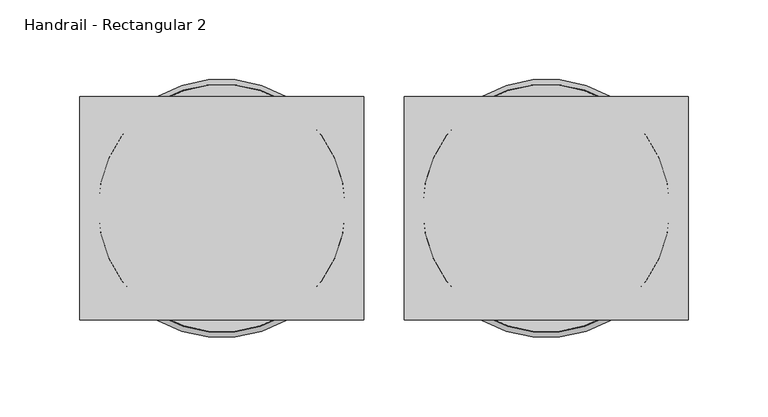
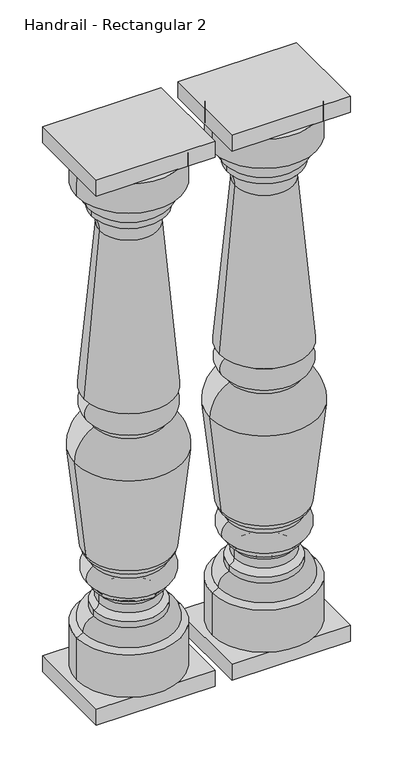
"""IFC4 building model written with IfcOpenShell, lengths in millimetres: railing geometry, Handrail - Rectangular 2."""

from ifc_helpers import new_model, si_unit, point, frame, origin, place, context, project, spatial, polyline, circle_curve, ellipse_curve, trimmed, outline, extrude, source, transform, mapped, element, save
from ifc_brep_helpers import plane_surface, cylinder_surface, revolved_surface, advanced_brep


def handrail_rectangular_2_8120b437(model_context):
    return source(origin(), model_context, "Body", "SolidModel", [
        advanced_brep(
        [(9662.0521895, -1691.0164768, 949.325), (9584.4909506, -1691.0164768, 949.325), (9739.6134284, -1691.0164768, 949.325), (9739.8396895, -1691.0164768, 136.525), (9584.2646895, -1691.0164768, 136.525), (9662.0521895, -1691.0164768, 136.525), (9739.8396895, -1691.0164768, 203.2), (9584.2646895, -1691.0164768, 203.2), (9730.2276556, -1691.0164768, 208.348485), (9593.8767235, -1691.0164768, 208.348485), (9714.4396895, -1691.0164768, 228.7310532), (9609.6646895, -1691.0164768, 228.7310532), (9714.4396895, -1691.0164768, 238.125), (9609.6646895, -1691.0164768, 238.125), (9706.8209727, -1691.0164768, 247.1598162), (9617.2834064, -1691.0164768, 247.1598162), (9706.8209727, -1691.0164768, 260.8401838), (9617.2834064, -1691.0164768, 260.8401838), (9714.4396895, -1691.0164768, 269.875), (9609.6646895, -1691.0164768, 269.875), (9714.4396895, -1691.0164768, 276.225), (9609.6646895, -1691.0164768, 276.225), (9715.2334395, -1691.0164768, 307.975), (9608.8709395, -1691.0164768, 307.975), (9715.2334395, -1691.0164768, 314.325), (9608.8709395, -1691.0164768, 314.325), (9726.0062243, -1691.0164768, 327.0157842), (9598.0981547, -1691.0164768, 327.0157842), (9743.093305, -1691.0164768, 481.3725887), (9581.0110741, -1691.0164768, 481.3725887), (9714.4396895, -1691.0164768, 528.6375), (9609.6646895, -1691.0164768, 528.6375), (9714.4396895, -1691.0164768, 534.9875), (9609.6646895, -1691.0164768, 534.9875), (9717.6146895, -1691.0164768, 569.9125), (9606.4896895, -1691.0164768, 569.9125), (9717.6146895, -1691.0164768, 573.0875), (9606.4896895, -1691.0164768, 573.0875), (9728.7271895, -1691.0164768, 577.85), (9595.3771895, -1691.0164768, 577.85), (9705.5486775, -1691.0164768, 836.3199218), (9618.5557016, -1691.0164768, 836.3199218), (9717.6146895, -1691.0164768, 863.6), (9606.4896895, -1691.0164768, 863.6), (9717.6146895, -1691.0164768, 873.125), (9606.4896895, -1691.0164768, 873.125), (9728.7271895, -1691.0164768, 900.1125), (9595.3771895, -1691.0164768, 900.1125), (9739.8396895, -1691.0164768, 903.2875), (9584.2646895, -1691.0164768, 903.2875)],
        [
            (0, 1),
            (1, 2, circle_curve(frame((9662.0521895, -1691.0164768, 949.325), z_axis=(0.0, 0.0, 1.0), x_axis=(-1.0, 0.0, 0.0)), 77.5612389)),
            (2, 0),
            (2, 1, circle_curve(frame((9662.0521895, -1691.0164768, 949.325), z_axis=(0.0, 0.0, 1.0), x_axis=(-1.0, 0.0, 0.0)), 77.5612389)),
            (3, 4, circle_curve(frame((9662.0521895, -1691.0164768, 136.525), z_axis=(0.0, 0.0, -1.0), x_axis=(-1.0, 0.0, 0.0)), 77.7875)),
            (4, 5),
            (5, 3),
            (4, 3, circle_curve(frame((9662.0521895, -1691.0164768, 136.525), z_axis=(0.0, 0.0, -1.0), x_axis=(-1.0, 0.0, 0.0)), 77.7875)),
            (6, 7, circle_curve(frame((9662.0521895, -1691.0164768, 203.2), z_axis=(0.0, 0.0, -1.0), x_axis=(-1.0, 0.0, 0.0)), 77.7875)),
            (7, 4),
            (3, 6),
            (7, 6, circle_curve(frame((9662.0521895, -1691.0164768, 203.2), z_axis=(0.0, 0.0, -1.0), x_axis=(-1.0, 0.0, 0.0)), 77.7875)),
            (8, 9, circle_curve(frame((9662.0521895, -1691.0164768, 208.348485), z_axis=(0.0, 0.0, -1.0), x_axis=(-1.0, 0.0, 0.0)), 68.175466)),
            (9, 7),
            (6, 8),
            (9, 8, circle_curve(frame((9662.0521895, -1691.0164768, 208.348485), z_axis=(0.0, 0.0, -1.0), x_axis=(-1.0, 0.0, 0.0)), 68.175466)),
            (10, 11, circle_curve(frame((9662.0521895, -1691.0164768, 228.7310532), z_axis=(0.0, 0.0, -1.0), x_axis=(-1.0, 0.0, 0.0)), 52.3875)),
            (11, 9, circle_curve(frame((9612.0397784, -1691.0164768, 210.5855331), z_axis=(0.0, -1.0, 0.0), x_axis=(1.0, 0.0, 0.0)), 18.3002991)),
            (8, 10, circle_curve(frame((9712.0646007, -1691.0164768, 210.5855331), z_axis=(0.0, -1.0, 0.0), x_axis=(-1.0, 0.0, 0.0)), 18.3002991)),
            (11, 10, circle_curve(frame((9662.0521895, -1691.0164768, 228.7310532), z_axis=(0.0, 0.0, -1.0), x_axis=(-1.0, 0.0, 0.0)), 52.3875)),
            (12, 13, circle_curve(frame((9662.0521895, -1691.0164768, 238.125), z_axis=(0.0, 0.0, -1.0), x_axis=(-1.0, 0.0, 0.0)), 52.3875)),
            (13, 11),
            (10, 12),
            (13, 12, circle_curve(frame((9662.0521895, -1691.0164768, 238.125), z_axis=(0.0, 0.0, -1.0), x_axis=(-1.0, 0.0, 0.0)), 52.3875)),
            (14, 15, circle_curve(frame((9662.0521895, -1691.0164768, 247.1598162), z_axis=(0.0, 0.0, -1.0), x_axis=(-1.0, 0.0, 0.0)), 44.7687831)),
            (15, 13, circle_curve(frame((9607.8793543, -1691.0164768, 247.3602005), z_axis=(0.0, 1.0, 0.0), x_axis=(1.0, 0.0, 0.0)), 9.4061868)),
            (12, 14, circle_curve(frame((9716.2250248, -1691.0164768, 247.3602005), z_axis=(0.0, 1.0, 0.0), x_axis=(-1.0, 0.0, 0.0)), 9.4061868)),
            (15, 14, circle_curve(frame((9662.0521895, -1691.0164768, 247.1598162), z_axis=(0.0, 0.0, -1.0), x_axis=(-1.0, 0.0, 0.0)), 44.7687831)),
            (16, 17, circle_curve(frame((9662.0521895, -1691.0164768, 260.8401838), z_axis=(0.0, 0.0, -1.0), x_axis=(-1.0, 0.0, 0.0)), 44.7687831)),
            (17, 15),
            (14, 16),
            (17, 16, circle_curve(frame((9662.0521895, -1691.0164768, 260.8401838), z_axis=(0.0, 0.0, -1.0), x_axis=(-1.0, 0.0, 0.0)), 44.7687831)),
            (18, 19, circle_curve(frame((9662.0521895, -1691.0164768, 269.875), z_axis=(0.0, 0.0, -1.0), x_axis=(-1.0, 0.0, 0.0)), 52.3875)),
            (19, 17, circle_curve(frame((9607.8793543, -1691.0164768, 260.6397995), z_axis=(0.0, 1.0, 0.0), x_axis=(1.0, 0.0, 0.0)), 9.4061868)),
            (16, 18, circle_curve(frame((9716.2250248, -1691.0164768, 260.6397995), z_axis=(0.0, 1.0, 0.0), x_axis=(-1.0, 0.0, 0.0)), 9.4061868)),
            (19, 18, circle_curve(frame((9662.0521895, -1691.0164768, 269.875), z_axis=(0.0, 0.0, -1.0), x_axis=(-1.0, 0.0, 0.0)), 52.3875)),
            (20, 21, circle_curve(frame((9662.0521895, -1691.0164768, 276.225), z_axis=(0.0, 0.0, -1.0), x_axis=(-1.0, 0.0, 0.0)), 52.3875)),
            (21, 19),
            (18, 20),
            (21, 20, circle_curve(frame((9662.0521895, -1691.0164768, 276.225), z_axis=(0.0, 0.0, -1.0), x_axis=(-1.0, 0.0, 0.0)), 52.3875)),
            (22, 23, circle_curve(frame((9662.0521895, -1691.0164768, 307.975), z_axis=(0.0, 0.0, -1.0), x_axis=(-1.0, 0.0, 0.0)), 53.18125)),
            (23, 21, circle_curve(frame((9615.2437772, -1691.0164768, 292.2493991), z_axis=(0.0, -1.0, 0.0), x_axis=(1.0, 0.0, 0.0)), 16.9678397)),
            (20, 22, circle_curve(frame((9708.8606019, -1691.0164768, 292.2493991), z_axis=(0.0, -1.0, 0.0), x_axis=(-1.0, 0.0, 0.0)), 16.9678397)),
            (23, 22, circle_curve(frame((9662.0521895, -1691.0164768, 307.975), z_axis=(0.0, 0.0, -1.0), x_axis=(-1.0, 0.0, 0.0)), 53.18125)),
            (24, 25, circle_curve(frame((9662.0521895, -1691.0164768, 314.325), z_axis=(0.0, 0.0, -1.0), x_axis=(-1.0, 0.0, 0.0)), 53.18125)),
            (25, 23),
            (22, 24),
            (25, 24, circle_curve(frame((9662.0521895, -1691.0164768, 314.325), z_axis=(0.0, 0.0, -1.0), x_axis=(-1.0, 0.0, 0.0)), 53.18125)),
            (26, 27, circle_curve(frame((9662.0521895, -1691.0164768, 327.0157842), z_axis=(0.0, 0.0, -1.0), x_axis=(-1.0, 0.0, 0.0)), 63.9540348)),
            (27, 25, circle_curve(frame((9618.704312, -1691.0164768, 333.5899445), z_axis=(0.0, -1.0, 0.0), x_axis=(1.0, 0.0, 0.0)), 21.6294545)),
            (24, 26, circle_curve(frame((9705.4000671, -1691.0164768, 333.5899445), z_axis=(0.0, -1.0, 0.0), x_axis=(-1.0, 0.0, 0.0)), 21.6294545)),
            (27, 26, circle_curve(frame((9662.0521895, -1691.0164768, 327.0157842), z_axis=(0.0, 0.0, -1.0), x_axis=(-1.0, 0.0, 0.0)), 63.9540348)),
            (28, 29, circle_curve(frame((9662.0521895, -1691.0164768, 481.3725887), z_axis=(0.0, 0.0, -1.0), x_axis=(-1.0, 0.0, 0.0)), 81.0411154)),
            (29, 27, circle_curve(frame((11075.3385198, -1691.0164768, 568.6683698), z_axis=(0.0, -1.0, 0.0), x_axis=(1.0, 0.0, 0.0)), 1496.8751012)),
            (26, 28, circle_curve(frame((8248.7658592, -1691.0164768, 568.6683698), z_axis=(0.0, -1.0, 0.0), x_axis=(-1.0, 0.0, 0.0)), 1496.8751012)),
            (29, 28, circle_curve(frame((9662.0521895, -1691.0164768, 481.3725887), z_axis=(0.0, 0.0, -1.0), x_axis=(-1.0, 0.0, 0.0)), 81.0411154)),
            (30, 31, circle_curve(frame((9662.0521895, -1691.0164768, 528.6375), z_axis=(0.0, 0.0, -1.0), x_axis=(-1.0, 0.0, 0.0)), 52.3875)),
            (31, 29, circle_curve(frame((9632.7638402, -1691.0164768, 482.3161407), z_axis=(0.0, -1.0, 0.0), x_axis=(1.0, 0.0, 0.0)), 51.7613668)),
            (28, 30, circle_curve(frame((9691.3405389, -1691.0164768, 482.3161407), z_axis=(0.0, -1.0, 0.0), x_axis=(-1.0, 0.0, 0.0)), 51.7613668)),
            (31, 30, circle_curve(frame((9662.0521895, -1691.0164768, 528.6375), z_axis=(0.0, 0.0, -1.0), x_axis=(-1.0, 0.0, 0.0)), 52.3875)),
            (32, 33, circle_curve(frame((9662.0521895, -1691.0164768, 534.9875), z_axis=(0.0, 0.0, -1.0), x_axis=(-1.0, 0.0, 0.0)), 52.3875)),
            (33, 31),
            (30, 32),
            (33, 32, circle_curve(frame((9662.0521895, -1691.0164768, 534.9875), z_axis=(0.0, 0.0, -1.0), x_axis=(-1.0, 0.0, 0.0)), 52.3875)),
            (34, 35, circle_curve(frame((9662.0521895, -1691.0164768, 569.9125), z_axis=(0.0, 0.0, -1.0), x_axis=(-1.0, 0.0, 0.0)), 55.5625)),
            (35, 33, circle_curve(frame((9614.7309419, -1691.0164768, 553.0548866), z_axis=(0.0, -1.0, 0.0), x_axis=(1.0, 0.0, 0.0)), 18.7642578)),
            (32, 34, circle_curve(frame((9709.3734372, -1691.0164768, 553.0548866), z_axis=(0.0, -1.0, 0.0), x_axis=(-1.0, 0.0, 0.0)), 18.7642578)),
            (35, 34, circle_curve(frame((9662.0521895, -1691.0164768, 569.9125), z_axis=(0.0, 0.0, -1.0), x_axis=(-1.0, 0.0, 0.0)), 55.5625)),
            (36, 37, circle_curve(frame((9662.0521895, -1691.0164768, 573.0875), z_axis=(0.0, 0.0, -1.0), x_axis=(-1.0, 0.0, 0.0)), 55.5625)),
            (37, 35),
            (34, 36),
            (37, 36, circle_curve(frame((9662.0521895, -1691.0164768, 573.0875), z_axis=(0.0, 0.0, -1.0), x_axis=(-1.0, 0.0, 0.0)), 55.5625)),
            (38, 39, circle_curve(frame((9662.0521895, -1691.0164768, 577.85), z_axis=(0.0, 0.0, -1.0), x_axis=(-1.0, 0.0, 0.0)), 66.675)),
            (39, 37),
            (36, 38),
            (39, 38, circle_curve(frame((9662.0521895, -1691.0164768, 577.85), z_axis=(0.0, 0.0, -1.0), x_axis=(-1.0, 0.0, 0.0)), 66.675)),
            (40, 41, circle_curve(frame((9662.0521895, -1691.0164768, 836.3199218), z_axis=(0.0, 0.0, -1.0), x_axis=(-1.0, 0.0, 0.0)), 43.4964879)),
            (41, 39, circle_curve(frame((7971.7192757, -1691.0164768, 853.7271544), z_axis=(0.0, 1.0, 0.0), x_axis=(1.0, 0.0, 0.0)), 1646.9284215)),
            (38, 40, circle_curve(frame((11352.3851034, -1691.0164768, 853.7271544), z_axis=(0.0, 1.0, 0.0), x_axis=(-1.0, 0.0, 0.0)), 1646.9284215)),
            (41, 40, circle_curve(frame((9662.0521895, -1691.0164768, 836.3199218), z_axis=(0.0, 0.0, -1.0), x_axis=(-1.0, 0.0, 0.0)), 43.4964879)),
            (42, 43, circle_curve(frame((9662.0521895, -1691.0164768, 863.6), z_axis=(0.0, 0.0, -1.0), x_axis=(-1.0, 0.0, 0.0)), 55.5625)),
            (43, 41, circle_curve(frame((9585.8515427, -1691.0164768, 838.1632773), z_axis=(0.0, 1.0, 0.0), x_axis=(1.0, 0.0, 0.0)), 32.7560676)),
            (40, 42, circle_curve(frame((9738.2528363, -1691.0164768, 838.1632773), z_axis=(0.0, 1.0, 0.0), x_axis=(-1.0, 0.0, 0.0)), 32.7560676)),
            (43, 42, circle_curve(frame((9662.0521895, -1691.0164768, 863.6), z_axis=(0.0, 0.0, -1.0), x_axis=(-1.0, 0.0, 0.0)), 55.5625)),
            (44, 45, circle_curve(frame((9662.0521895, -1691.0164768, 873.125), z_axis=(0.0, 0.0, -1.0), x_axis=(-1.0, 0.0, 0.0)), 55.5625)),
            (45, 43),
            (42, 44),
            (45, 44, circle_curve(frame((9662.0521895, -1691.0164768, 873.125), z_axis=(0.0, 0.0, -1.0), x_axis=(-1.0, 0.0, 0.0)), 55.5625)),
            (46, 47, circle_curve(frame((9662.0521895, -1691.0164768, 900.1125), z_axis=(0.0, 0.0, -1.0), x_axis=(-1.0, 0.0, 0.0)), 66.675)),
            (47, 45, circle_curve(frame((9624.7374113, -1691.0164768, 896.4203854), z_axis=(0.0, -1.0, 0.0), x_axis=(1.0, 0.0, 0.0)), 29.5914571)),
            (44, 46, circle_curve(frame((9699.3669678, -1691.0164768, 896.4203854), z_axis=(0.0, -1.0, 0.0), x_axis=(-1.0, 0.0, 0.0)), 29.5914571)),
            (47, 46, circle_curve(frame((9662.0521895, -1691.0164768, 900.1125), z_axis=(0.0, 0.0, -1.0), x_axis=(-1.0, 0.0, 0.0)), 66.675)),
            (48, 49, circle_curve(frame((9662.0521895, -1691.0164768, 903.2875), z_axis=(0.0, 0.0, -1.0), x_axis=(-1.0, 0.0, 0.0)), 77.7875)),
            (49, 47),
            (46, 48),
            (49, 48, circle_curve(frame((9662.0521895, -1691.0164768, 903.2875), z_axis=(0.0, 0.0, -1.0), x_axis=(-1.0, 0.0, 0.0)), 77.7875)),
            (1, 49),
            (48, 2),
        ],
        [
            plane_surface(frame((9662.0521895, -1691.0164768, 949.325), z_axis=(0.0, 0.0, 1.0), x_axis=(-1.0, 0.0, 0.0))),
            plane_surface(frame((9662.0521895, -1691.0164768, 136.525), z_axis=(0.0, 0.0, -1.0), x_axis=(-1.0, 0.0, 0.0))),
            cylinder_surface(frame((9662.0521895, -1691.0164768, 1019.175), z_axis=(0.0, 0.0, 1.0), x_axis=(-1.0, 0.0, 0.0)), 77.7875),
            revolved_surface(polyline([(9584.2646895, -1691.0164768, 203.2), (9593.8767235, -1691.0164768, 208.348485)]), (9662.0521895, -1691.0164768, 1019.175), (0.0, 0.0, 1.0)),
            revolved_surface(trimmed(ellipse_curve(frame((9612.0397784, -1691.0164768, 210.5855331), z_axis=(0.0, 1.0, 0.0), x_axis=(1.0, 0.0, 0.0)), 18.3002991, 18.3002991), [point((9593.8767235, -1691.0164768, 208.348485))], [point((9609.6646895, -1691.0164768, 228.7310532))], True, "CARTESIAN"), (9662.0521895, -1691.0164768, 1019.175), (0.0, 0.0, 1.0)),
            cylinder_surface(frame((9662.0521895, -1691.0164768, 1019.175), z_axis=(0.0, 0.0, 1.0), x_axis=(-1.0, 0.0, 0.0)), 52.3875),
            revolved_surface(trimmed(ellipse_curve(frame((9607.8793543, -1691.0164768, 247.3602005), z_axis=(0.0, -1.0, 0.0), x_axis=(1.0, 0.0, 0.0)), 9.4061868, 9.4061868), [point((9609.6646895, -1691.0164768, 238.125))], [point((9617.2834064, -1691.0164768, 247.1598162))], True, "CARTESIAN"), (9662.0521895, -1691.0164768, 1019.175), (0.0, 0.0, 1.0)),
            cylinder_surface(frame((9662.0521895, -1691.0164768, 1019.175), z_axis=(0.0, 0.0, 1.0), x_axis=(-1.0, 0.0, 0.0)), 44.7687831),
            revolved_surface(trimmed(ellipse_curve(frame((9607.8793543, -1691.0164768, 260.6397995), z_axis=(0.0, -1.0, 0.0), x_axis=(1.0, 0.0, 0.0)), 9.4061868, 9.4061868), [point((9617.2834064, -1691.0164768, 260.8401838))], [point((9609.6646895, -1691.0164768, 269.875))], True, "CARTESIAN"), (9662.0521895, -1691.0164768, 1019.175), (0.0, 0.0, 1.0)),
            revolved_surface(trimmed(ellipse_curve(frame((9615.2437772, -1691.0164768, 292.2493991), z_axis=(0.0, 1.0, 0.0), x_axis=(1.0, 0.0, 0.0)), 16.9678397, 16.9678397), [point((9609.6646895, -1691.0164768, 276.225))], [point((9608.8709395, -1691.0164768, 307.975))], True, "CARTESIAN"), (9662.0521895, -1691.0164768, 1019.175), (0.0, 0.0, 1.0)),
            cylinder_surface(frame((9662.0521895, -1691.0164768, 1019.175), z_axis=(0.0, 0.0, 1.0), x_axis=(-1.0, 0.0, 0.0)), 53.18125),
            revolved_surface(trimmed(ellipse_curve(frame((9618.704312, -1691.0164768, 333.5899445), z_axis=(0.0, 1.0, 0.0), x_axis=(1.0, 0.0, 0.0)), 21.6294545, 21.6294545), [point((9608.8709395, -1691.0164768, 314.325))], [point((9598.0981547, -1691.0164768, 327.0157842))], True, "CARTESIAN"), (9662.0521895, -1691.0164768, 1019.175), (0.0, 0.0, 1.0)),
            revolved_surface(trimmed(ellipse_curve(frame((11075.3385198, -1691.0164768, 568.6683698), z_axis=(0.0, 1.0, 0.0), x_axis=(1.0, 0.0, 0.0)), 1496.8751012, 1496.8751012), [point((9598.0981547, -1691.0164768, 327.0157842))], [point((9581.0110741, -1691.0164768, 481.3725887))], True, "CARTESIAN"), (9662.0521895, -1691.0164768, 1019.175), (0.0, 0.0, 1.0)),
            revolved_surface(trimmed(ellipse_curve(frame((9632.7638402, -1691.0164768, 482.3161407), z_axis=(0.0, 1.0, 0.0), x_axis=(1.0, 0.0, 0.0)), 51.7613668, 51.7613668), [point((9581.0110741, -1691.0164768, 481.3725887))], [point((9609.6646895, -1691.0164768, 528.6375))], True, "CARTESIAN"), (9662.0521895, -1691.0164768, 1019.175), (0.0, 0.0, 1.0)),
            revolved_surface(trimmed(ellipse_curve(frame((9614.7309419, -1691.0164768, 553.0548866), z_axis=(0.0, 1.0, 0.0), x_axis=(1.0, 0.0, 0.0)), 18.7642578, 18.7642578), [point((9609.6646895, -1691.0164768, 534.9875))], [point((9606.4896895, -1691.0164768, 569.9125))], True, "CARTESIAN"), (9662.0521895, -1691.0164768, 1019.175), (0.0, 0.0, 1.0)),
            cylinder_surface(frame((9662.0521895, -1691.0164768, 1019.175), z_axis=(0.0, 0.0, 1.0), x_axis=(-1.0, 0.0, 0.0)), 55.5625),
            revolved_surface(polyline([(9606.4896895, -1691.0164768, 573.0875), (9595.3771895, -1691.0164768, 577.85)]), (9662.0521895, -1691.0164768, 1019.175), (0.0, 0.0, 1.0)),
            revolved_surface(trimmed(ellipse_curve(frame((7971.7192757, -1691.0164768, 853.7271544), z_axis=(0.0, -1.0, 0.0), x_axis=(1.0, 0.0, 0.0)), 1646.9284215, 1646.9284215), [point((9595.3771895, -1691.0164768, 577.85))], [point((9618.5557016, -1691.0164768, 836.3199218))], True, "CARTESIAN"), (9662.0521895, -1691.0164768, 1019.175), (0.0, 0.0, 1.0)),
            revolved_surface(trimmed(ellipse_curve(frame((9585.8515427, -1691.0164768, 838.1632773), z_axis=(0.0, -1.0, 0.0), x_axis=(1.0, 0.0, 0.0)), 32.7560676, 32.7560676), [point((9618.5557016, -1691.0164768, 836.3199218))], [point((9606.4896895, -1691.0164768, 863.6))], True, "CARTESIAN"), (9662.0521895, -1691.0164768, 1019.175), (0.0, 0.0, 1.0)),
            revolved_surface(trimmed(ellipse_curve(frame((9624.7374113, -1691.0164768, 896.4203854), z_axis=(0.0, 1.0, 0.0), x_axis=(1.0, 0.0, 0.0)), 29.5914571, 29.5914571), [point((9606.4896895, -1691.0164768, 873.125))], [point((9595.3771895, -1691.0164768, 900.1125))], True, "CARTESIAN"), (9662.0521895, -1691.0164768, 1019.175), (0.0, 0.0, 1.0)),
            revolved_surface(polyline([(9595.3771895, -1691.0164768, 900.1125), (9584.2646895, -1691.0164768, 903.2875)]), (9662.0521895, -1691.0164768, 1019.175), (0.0, 0.0, 1.0)),
            revolved_surface(polyline([(9584.2646895, -1691.0164768, 903.2875), (9584.4909506, -1691.0164768, 949.325)]), (9662.0521895, -1691.0164768, 1019.175), (0.0, 0.0, 1.0)),
        ],
        [
            (0, [[1, 2, 3]]),
            (0, [[-3, 4, -1]]),
            (1, [[5, 6, 7]]),
            (1, [[8, -7, -6]]),
            (2, [[9, 10, -5, 11]]),
            (2, [[12, -11, -8, -10]]),
            (3, [[13, 14, -9, 15]]),
            (3, [[16, -15, -12, -14]]),
            (4, [[17, 18, -13, 19]]),
            (4, [[20, -19, -16, -18]]),
            (5, [[21, 22, -17, 23]]),
            (5, [[24, -23, -20, -22]]),
            (6, [[25, 26, -21, 27]]),
            (6, [[28, -27, -24, -26]]),
            (7, [[29, 30, -25, 31]]),
            (7, [[32, -31, -28, -30]]),
            (8, [[33, 34, -29, 35]]),
            (8, [[36, -35, -32, -34]]),
            (5, [[37, 38, -33, 39]]),
            (5, [[40, -39, -36, -38]]),
            (9, [[41, 42, -37, 43]]),
            (9, [[44, -43, -40, -42]]),
            (10, [[45, 46, -41, 47]]),
            (10, [[48, -47, -44, -46]]),
            (11, [[49, 50, -45, 51]]),
            (11, [[52, -51, -48, -50]]),
            (12, [[53, 54, -49, 55]]),
            (12, [[56, -55, -52, -54]]),
            (13, [[57, 58, -53, 59]]),
            (13, [[60, -59, -56, -58]]),
            (5, [[61, 62, -57, 63]]),
            (5, [[64, -63, -60, -62]]),
            (14, [[65, 66, -61, 67]]),
            (14, [[68, -67, -64, -66]]),
            (15, [[69, 70, -65, 71]]),
            (15, [[72, -71, -68, -70]]),
            (16, [[73, 74, -69, 75]]),
            (16, [[76, -75, -72, -74]]),
            (17, [[77, 78, -73, 79]]),
            (17, [[80, -79, -76, -78]]),
            (18, [[81, 82, -77, 83]]),
            (18, [[84, -83, -80, -82]]),
            (15, [[85, 86, -81, 87]]),
            (15, [[88, -87, -84, -86]]),
            (19, [[89, 90, -85, 91]]),
            (19, [[92, -91, -88, -90]]),
            (20, [[93, 94, -89, 95]]),
            (20, [[96, -95, -92, -94]]),
            (21, [[-2, 97, -93, 98]]),
            (21, [[-4, -98, -96, -97]]),
        ],
    ),
        extrude(outline(polyline([(9573.1521895, -1760.8664768), (9573.1521895, -1621.1664768), (9750.9521895, -1621.1664768), (9750.9521895, -1760.8664768), (9573.1521895, -1760.8664768)])), frame((0.0, 0.0, 111.125), z_axis=(0.0, 0.0, 1.0), x_axis=(1.0, 0.0, 0.0)), (0.0, 0.0, 1.0), 25.4),
        extrude(outline(polyline([(9573.1521895, -1621.1664768), (9750.9521895, -1621.1664768), (9750.9521895, -1760.8664768), (9573.1521895, -1760.8664768), (9573.1521895, -1621.1664768)])), frame((0.0, 0.0, 949.325), z_axis=(0.0, 0.0, 1.0), x_axis=(1.0, 0.0, 0.0)), (0.0, 0.0, 1.0), 25.4),
        advanced_brep(
        [(9458.8521895, -1691.0164768, 949.325), (9381.2909506, -1691.0164768, 949.325), (9536.4134284, -1691.0164768, 949.325), (9536.6396895, -1691.0164768, 136.525), (9381.0646895, -1691.0164768, 136.525), (9458.8521895, -1691.0164768, 136.525), (9536.6396895, -1691.0164768, 203.2), (9381.0646895, -1691.0164768, 203.2), (9527.0276556, -1691.0164768, 208.348485), (9390.6767235, -1691.0164768, 208.348485), (9511.2396895, -1691.0164768, 228.7310532), (9406.4646895, -1691.0164768, 228.7310532), (9511.2396895, -1691.0164768, 238.125), (9406.4646895, -1691.0164768, 238.125), (9503.6209727, -1691.0164768, 247.1598162), (9414.0834064, -1691.0164768, 247.1598162), (9503.6209727, -1691.0164768, 260.8401838), (9414.0834064, -1691.0164768, 260.8401838), (9511.2396895, -1691.0164768, 269.875), (9406.4646895, -1691.0164768, 269.875), (9511.2396895, -1691.0164768, 276.225), (9406.4646895, -1691.0164768, 276.225), (9512.0334395, -1691.0164768, 307.975), (9405.6709395, -1691.0164768, 307.975), (9512.0334395, -1691.0164768, 314.325), (9405.6709395, -1691.0164768, 314.325), (9522.8062243, -1691.0164768, 327.0157842), (9394.8981547, -1691.0164768, 327.0157842), (9539.893305, -1691.0164768, 481.3725887), (9377.8110741, -1691.0164768, 481.3725887), (9511.2396895, -1691.0164768, 528.6375), (9406.4646895, -1691.0164768, 528.6375), (9511.2396895, -1691.0164768, 534.9875), (9406.4646895, -1691.0164768, 534.9875), (9514.4146895, -1691.0164768, 569.9125), (9403.2896895, -1691.0164768, 569.9125), (9514.4146895, -1691.0164768, 573.0875), (9403.2896895, -1691.0164768, 573.0875), (9525.5271895, -1691.0164768, 577.85), (9392.1771895, -1691.0164768, 577.85), (9502.3486775, -1691.0164768, 836.3199218), (9415.3557016, -1691.0164768, 836.3199218), (9514.4146895, -1691.0164768, 863.6), (9403.2896895, -1691.0164768, 863.6), (9514.4146895, -1691.0164768, 873.125), (9403.2896895, -1691.0164768, 873.125), (9525.5271895, -1691.0164768, 900.1125), (9392.1771895, -1691.0164768, 900.1125), (9536.6396895, -1691.0164768, 903.2875), (9381.0646895, -1691.0164768, 903.2875)],
        [
            (0, 1),
            (1, 2, circle_curve(frame((9458.8521895, -1691.0164768, 949.325), z_axis=(0.0, 0.0, 1.0), x_axis=(-1.0, 0.0, 0.0)), 77.5612389)),
            (2, 0),
            (2, 1, circle_curve(frame((9458.8521895, -1691.0164768, 949.325), z_axis=(0.0, 0.0, 1.0), x_axis=(-1.0, 0.0, 0.0)), 77.5612389)),
            (3, 4, circle_curve(frame((9458.8521895, -1691.0164768, 136.525), z_axis=(0.0, 0.0, -1.0), x_axis=(-1.0, 0.0, 0.0)), 77.7875)),
            (4, 5),
            (5, 3),
            (4, 3, circle_curve(frame((9458.8521895, -1691.0164768, 136.525), z_axis=(0.0, 0.0, -1.0), x_axis=(-1.0, 0.0, 0.0)), 77.7875)),
            (6, 7, circle_curve(frame((9458.8521895, -1691.0164768, 203.2), z_axis=(0.0, 0.0, -1.0), x_axis=(-1.0, 0.0, 0.0)), 77.7875)),
            (7, 4),
            (3, 6),
            (7, 6, circle_curve(frame((9458.8521895, -1691.0164768, 203.2), z_axis=(0.0, 0.0, -1.0), x_axis=(-1.0, 0.0, 0.0)), 77.7875)),
            (8, 9, circle_curve(frame((9458.8521895, -1691.0164768, 208.348485), z_axis=(0.0, 0.0, -1.0), x_axis=(-1.0, 0.0, 0.0)), 68.175466)),
            (9, 7),
            (6, 8),
            (9, 8, circle_curve(frame((9458.8521895, -1691.0164768, 208.348485), z_axis=(0.0, 0.0, -1.0), x_axis=(-1.0, 0.0, 0.0)), 68.175466)),
            (10, 11, circle_curve(frame((9458.8521895, -1691.0164768, 228.7310532), z_axis=(0.0, 0.0, -1.0), x_axis=(-1.0, 0.0, 0.0)), 52.3875)),
            (11, 9, circle_curve(frame((9408.8397784, -1691.0164768, 210.5855331), z_axis=(0.0, -1.0, 0.0), x_axis=(1.0, 0.0, 0.0)), 18.3002991)),
            (8, 10, circle_curve(frame((9508.8646007, -1691.0164768, 210.5855331), z_axis=(0.0, -1.0, 0.0), x_axis=(-1.0, 0.0, 0.0)), 18.3002991)),
            (11, 10, circle_curve(frame((9458.8521895, -1691.0164768, 228.7310532), z_axis=(0.0, 0.0, -1.0), x_axis=(-1.0, 0.0, 0.0)), 52.3875)),
            (12, 13, circle_curve(frame((9458.8521895, -1691.0164768, 238.125), z_axis=(0.0, 0.0, -1.0), x_axis=(-1.0, 0.0, 0.0)), 52.3875)),
            (13, 11),
            (10, 12),
            (13, 12, circle_curve(frame((9458.8521895, -1691.0164768, 238.125), z_axis=(0.0, 0.0, -1.0), x_axis=(-1.0, 0.0, 0.0)), 52.3875)),
            (14, 15, circle_curve(frame((9458.8521895, -1691.0164768, 247.1598162), z_axis=(0.0, 0.0, -1.0), x_axis=(-1.0, 0.0, 0.0)), 44.7687831)),
            (15, 13, circle_curve(frame((9404.6793543, -1691.0164768, 247.3602005), z_axis=(0.0, 1.0, 0.0), x_axis=(1.0, 0.0, 0.0)), 9.4061868)),
            (12, 14, circle_curve(frame((9513.0250248, -1691.0164768, 247.3602005), z_axis=(0.0, 1.0, 0.0), x_axis=(-1.0, 0.0, 0.0)), 9.4061868)),
            (15, 14, circle_curve(frame((9458.8521895, -1691.0164768, 247.1598162), z_axis=(0.0, 0.0, -1.0), x_axis=(-1.0, 0.0, 0.0)), 44.7687831)),
            (16, 17, circle_curve(frame((9458.8521895, -1691.0164768, 260.8401838), z_axis=(0.0, 0.0, -1.0), x_axis=(-1.0, 0.0, 0.0)), 44.7687831)),
            (17, 15),
            (14, 16),
            (17, 16, circle_curve(frame((9458.8521895, -1691.0164768, 260.8401838), z_axis=(0.0, 0.0, -1.0), x_axis=(-1.0, 0.0, 0.0)), 44.7687831)),
            (18, 19, circle_curve(frame((9458.8521895, -1691.0164768, 269.875), z_axis=(0.0, 0.0, -1.0), x_axis=(-1.0, 0.0, 0.0)), 52.3875)),
            (19, 17, circle_curve(frame((9404.6793543, -1691.0164768, 260.6397995), z_axis=(0.0, 1.0, 0.0), x_axis=(1.0, 0.0, 0.0)), 9.4061868)),
            (16, 18, circle_curve(frame((9513.0250248, -1691.0164768, 260.6397995), z_axis=(0.0, 1.0, 0.0), x_axis=(-1.0, 0.0, 0.0)), 9.4061868)),
            (19, 18, circle_curve(frame((9458.8521895, -1691.0164768, 269.875), z_axis=(0.0, 0.0, -1.0), x_axis=(-1.0, 0.0, 0.0)), 52.3875)),
            (20, 21, circle_curve(frame((9458.8521895, -1691.0164768, 276.225), z_axis=(0.0, 0.0, -1.0), x_axis=(-1.0, 0.0, 0.0)), 52.3875)),
            (21, 19),
            (18, 20),
            (21, 20, circle_curve(frame((9458.8521895, -1691.0164768, 276.225), z_axis=(0.0, 0.0, -1.0), x_axis=(-1.0, 0.0, 0.0)), 52.3875)),
            (22, 23, circle_curve(frame((9458.8521895, -1691.0164768, 307.975), z_axis=(0.0, 0.0, -1.0), x_axis=(-1.0, 0.0, 0.0)), 53.18125)),
            (23, 21, circle_curve(frame((9412.0437772, -1691.0164768, 292.2493991), z_axis=(0.0, -1.0, 0.0), x_axis=(1.0, 0.0, 0.0)), 16.9678397)),
            (20, 22, circle_curve(frame((9505.6606019, -1691.0164768, 292.2493991), z_axis=(0.0, -1.0, 0.0), x_axis=(-1.0, 0.0, 0.0)), 16.9678397)),
            (23, 22, circle_curve(frame((9458.8521895, -1691.0164768, 307.975), z_axis=(0.0, 0.0, -1.0), x_axis=(-1.0, 0.0, 0.0)), 53.18125)),
            (24, 25, circle_curve(frame((9458.8521895, -1691.0164768, 314.325), z_axis=(0.0, 0.0, -1.0), x_axis=(-1.0, 0.0, 0.0)), 53.18125)),
            (25, 23),
            (22, 24),
            (25, 24, circle_curve(frame((9458.8521895, -1691.0164768, 314.325), z_axis=(0.0, 0.0, -1.0), x_axis=(-1.0, 0.0, 0.0)), 53.18125)),
            (26, 27, circle_curve(frame((9458.8521895, -1691.0164768, 327.0157842), z_axis=(0.0, 0.0, -1.0), x_axis=(-1.0, 0.0, 0.0)), 63.9540348)),
            (27, 25, circle_curve(frame((9415.504312, -1691.0164768, 333.5899445), z_axis=(0.0, -1.0, 0.0), x_axis=(1.0, 0.0, 0.0)), 21.6294545)),
            (24, 26, circle_curve(frame((9502.2000671, -1691.0164768, 333.5899445), z_axis=(0.0, -1.0, 0.0), x_axis=(-1.0, 0.0, 0.0)), 21.6294545)),
            (27, 26, circle_curve(frame((9458.8521895, -1691.0164768, 327.0157842), z_axis=(0.0, 0.0, -1.0), x_axis=(-1.0, 0.0, 0.0)), 63.9540348)),
            (28, 29, circle_curve(frame((9458.8521895, -1691.0164768, 481.3725887), z_axis=(0.0, 0.0, -1.0), x_axis=(-1.0, 0.0, 0.0)), 81.0411154)),
            (29, 27, circle_curve(frame((10872.1385198, -1691.0164768, 568.6683698), z_axis=(0.0, -1.0, 0.0), x_axis=(1.0, 0.0, 0.0)), 1496.8751012)),
            (26, 28, circle_curve(frame((8045.5658592, -1691.0164768, 568.6683698), z_axis=(0.0, -1.0, 0.0), x_axis=(-1.0, 0.0, 0.0)), 1496.8751012)),
            (29, 28, circle_curve(frame((9458.8521895, -1691.0164768, 481.3725887), z_axis=(0.0, 0.0, -1.0), x_axis=(-1.0, 0.0, 0.0)), 81.0411154)),
            (30, 31, circle_curve(frame((9458.8521895, -1691.0164768, 528.6375), z_axis=(0.0, 0.0, -1.0), x_axis=(-1.0, 0.0, 0.0)), 52.3875)),
            (31, 29, circle_curve(frame((9429.5638402, -1691.0164768, 482.3161407), z_axis=(0.0, -1.0, 0.0), x_axis=(1.0, 0.0, 0.0)), 51.7613668)),
            (28, 30, circle_curve(frame((9488.1405389, -1691.0164768, 482.3161407), z_axis=(0.0, -1.0, 0.0), x_axis=(-1.0, 0.0, 0.0)), 51.7613668)),
            (31, 30, circle_curve(frame((9458.8521895, -1691.0164768, 528.6375), z_axis=(0.0, 0.0, -1.0), x_axis=(-1.0, 0.0, 0.0)), 52.3875)),
            (32, 33, circle_curve(frame((9458.8521895, -1691.0164768, 534.9875), z_axis=(0.0, 0.0, -1.0), x_axis=(-1.0, 0.0, 0.0)), 52.3875)),
            (33, 31),
            (30, 32),
            (33, 32, circle_curve(frame((9458.8521895, -1691.0164768, 534.9875), z_axis=(0.0, 0.0, -1.0), x_axis=(-1.0, 0.0, 0.0)), 52.3875)),
            (34, 35, circle_curve(frame((9458.8521895, -1691.0164768, 569.9125), z_axis=(0.0, 0.0, -1.0), x_axis=(-1.0, 0.0, 0.0)), 55.5625)),
            (35, 33, circle_curve(frame((9411.5309419, -1691.0164768, 553.0548866), z_axis=(0.0, -1.0, 0.0), x_axis=(1.0, 0.0, 0.0)), 18.7642578)),
            (32, 34, circle_curve(frame((9506.1734372, -1691.0164768, 553.0548866), z_axis=(0.0, -1.0, 0.0), x_axis=(-1.0, 0.0, 0.0)), 18.7642578)),
            (35, 34, circle_curve(frame((9458.8521895, -1691.0164768, 569.9125), z_axis=(0.0, 0.0, -1.0), x_axis=(-1.0, 0.0, 0.0)), 55.5625)),
            (36, 37, circle_curve(frame((9458.8521895, -1691.0164768, 573.0875), z_axis=(0.0, 0.0, -1.0), x_axis=(-1.0, 0.0, 0.0)), 55.5625)),
            (37, 35),
            (34, 36),
            (37, 36, circle_curve(frame((9458.8521895, -1691.0164768, 573.0875), z_axis=(0.0, 0.0, -1.0), x_axis=(-1.0, 0.0, 0.0)), 55.5625)),
            (38, 39, circle_curve(frame((9458.8521895, -1691.0164768, 577.85), z_axis=(0.0, 0.0, -1.0), x_axis=(-1.0, 0.0, 0.0)), 66.675)),
            (39, 37),
            (36, 38),
            (39, 38, circle_curve(frame((9458.8521895, -1691.0164768, 577.85), z_axis=(0.0, 0.0, -1.0), x_axis=(-1.0, 0.0, 0.0)), 66.675)),
            (40, 41, circle_curve(frame((9458.8521895, -1691.0164768, 836.3199218), z_axis=(0.0, 0.0, -1.0), x_axis=(-1.0, 0.0, 0.0)), 43.4964879)),
            (41, 39, circle_curve(frame((7768.5192757, -1691.0164768, 853.7271544), z_axis=(0.0, 1.0, 0.0), x_axis=(1.0, 0.0, 0.0)), 1646.9284215)),
            (38, 40, circle_curve(frame((11149.1851034, -1691.0164768, 853.7271544), z_axis=(0.0, 1.0, 0.0), x_axis=(-1.0, 0.0, 0.0)), 1646.9284215)),
            (41, 40, circle_curve(frame((9458.8521895, -1691.0164768, 836.3199218), z_axis=(0.0, 0.0, -1.0), x_axis=(-1.0, 0.0, 0.0)), 43.4964879)),
            (42, 43, circle_curve(frame((9458.8521895, -1691.0164768, 863.6), z_axis=(0.0, 0.0, -1.0), x_axis=(-1.0, 0.0, 0.0)), 55.5625)),
            (43, 41, circle_curve(frame((9382.6515427, -1691.0164768, 838.1632773), z_axis=(0.0, 1.0, 0.0), x_axis=(1.0, 0.0, 0.0)), 32.7560676)),
            (40, 42, circle_curve(frame((9535.0528363, -1691.0164768, 838.1632773), z_axis=(0.0, 1.0, 0.0), x_axis=(-1.0, 0.0, 0.0)), 32.7560676)),
            (43, 42, circle_curve(frame((9458.8521895, -1691.0164768, 863.6), z_axis=(0.0, 0.0, -1.0), x_axis=(-1.0, 0.0, 0.0)), 55.5625)),
            (44, 45, circle_curve(frame((9458.8521895, -1691.0164768, 873.125), z_axis=(0.0, 0.0, -1.0), x_axis=(-1.0, 0.0, 0.0)), 55.5625)),
            (45, 43),
            (42, 44),
            (45, 44, circle_curve(frame((9458.8521895, -1691.0164768, 873.125), z_axis=(0.0, 0.0, -1.0), x_axis=(-1.0, 0.0, 0.0)), 55.5625)),
            (46, 47, circle_curve(frame((9458.8521895, -1691.0164768, 900.1125), z_axis=(0.0, 0.0, -1.0), x_axis=(-1.0, 0.0, 0.0)), 66.675)),
            (47, 45, circle_curve(frame((9421.5374113, -1691.0164768, 896.4203854), z_axis=(0.0, -1.0, 0.0), x_axis=(1.0, 0.0, 0.0)), 29.5914571)),
            (44, 46, circle_curve(frame((9496.1669678, -1691.0164768, 896.4203854), z_axis=(0.0, -1.0, 0.0), x_axis=(-1.0, 0.0, 0.0)), 29.5914571)),
            (47, 46, circle_curve(frame((9458.8521895, -1691.0164768, 900.1125), z_axis=(0.0, 0.0, -1.0), x_axis=(-1.0, 0.0, 0.0)), 66.675)),
            (48, 49, circle_curve(frame((9458.8521895, -1691.0164768, 903.2875), z_axis=(0.0, 0.0, -1.0), x_axis=(-1.0, 0.0, 0.0)), 77.7875)),
            (49, 47),
            (46, 48),
            (49, 48, circle_curve(frame((9458.8521895, -1691.0164768, 903.2875), z_axis=(0.0, 0.0, -1.0), x_axis=(-1.0, 0.0, 0.0)), 77.7875)),
            (1, 49),
            (48, 2),
        ],
        [
            plane_surface(frame((9458.8521895, -1691.0164768, 949.325), z_axis=(0.0, 0.0, 1.0), x_axis=(-1.0, 0.0, 0.0))),
            plane_surface(frame((9458.8521895, -1691.0164768, 136.525), z_axis=(0.0, 0.0, -1.0), x_axis=(-1.0, 0.0, 0.0))),
            cylinder_surface(frame((9458.8521895, -1691.0164768, 1019.175), z_axis=(0.0, 0.0, 1.0), x_axis=(-1.0, 0.0, 0.0)), 77.7875),
            revolved_surface(polyline([(9381.0646895, -1691.0164768, 203.2), (9390.6767235, -1691.0164768, 208.348485)]), (9458.8521895, -1691.0164768, 1019.175), (0.0, 0.0, 1.0)),
            revolved_surface(trimmed(ellipse_curve(frame((9408.8397784, -1691.0164768, 210.5855331), z_axis=(0.0, 1.0, 0.0), x_axis=(1.0, 0.0, 0.0)), 18.3002991, 18.3002991), [point((9390.6767235, -1691.0164768, 208.348485))], [point((9406.4646895, -1691.0164768, 228.7310532))], True, "CARTESIAN"), (9458.8521895, -1691.0164768, 1019.175), (0.0, 0.0, 1.0)),
            cylinder_surface(frame((9458.8521895, -1691.0164768, 1019.175), z_axis=(0.0, 0.0, 1.0), x_axis=(-1.0, 0.0, 0.0)), 52.3875),
            revolved_surface(trimmed(ellipse_curve(frame((9404.6793543, -1691.0164768, 247.3602005), z_axis=(0.0, -1.0, 0.0), x_axis=(1.0, 0.0, 0.0)), 9.4061868, 9.4061868), [point((9406.4646895, -1691.0164768, 238.125))], [point((9414.0834064, -1691.0164768, 247.1598162))], True, "CARTESIAN"), (9458.8521895, -1691.0164768, 1019.175), (0.0, 0.0, 1.0)),
            cylinder_surface(frame((9458.8521895, -1691.0164768, 1019.175), z_axis=(0.0, 0.0, 1.0), x_axis=(-1.0, 0.0, 0.0)), 44.7687831),
            revolved_surface(trimmed(ellipse_curve(frame((9404.6793543, -1691.0164768, 260.6397995), z_axis=(0.0, -1.0, 0.0), x_axis=(1.0, 0.0, 0.0)), 9.4061868, 9.4061868), [point((9414.0834064, -1691.0164768, 260.8401838))], [point((9406.4646895, -1691.0164768, 269.875))], True, "CARTESIAN"), (9458.8521895, -1691.0164768, 1019.175), (0.0, 0.0, 1.0)),
            revolved_surface(trimmed(ellipse_curve(frame((9412.0437772, -1691.0164768, 292.2493991), z_axis=(0.0, 1.0, 0.0), x_axis=(1.0, 0.0, 0.0)), 16.9678397, 16.9678397), [point((9406.4646895, -1691.0164768, 276.225))], [point((9405.6709395, -1691.0164768, 307.975))], True, "CARTESIAN"), (9458.8521895, -1691.0164768, 1019.175), (0.0, 0.0, 1.0)),
            cylinder_surface(frame((9458.8521895, -1691.0164768, 1019.175), z_axis=(0.0, 0.0, 1.0), x_axis=(-1.0, 0.0, 0.0)), 53.18125),
            revolved_surface(trimmed(ellipse_curve(frame((9415.504312, -1691.0164768, 333.5899445), z_axis=(0.0, 1.0, 0.0), x_axis=(1.0, 0.0, 0.0)), 21.6294545, 21.6294545), [point((9405.6709395, -1691.0164768, 314.325))], [point((9394.8981547, -1691.0164768, 327.0157842))], True, "CARTESIAN"), (9458.8521895, -1691.0164768, 1019.175), (0.0, 0.0, 1.0)),
            revolved_surface(trimmed(ellipse_curve(frame((10872.1385198, -1691.0164768, 568.6683698), z_axis=(0.0, 1.0, 0.0), x_axis=(1.0, 0.0, 0.0)), 1496.8751012, 1496.8751012), [point((9394.8981547, -1691.0164768, 327.0157842))], [point((9377.8110741, -1691.0164768, 481.3725887))], True, "CARTESIAN"), (9458.8521895, -1691.0164768, 1019.175), (0.0, 0.0, 1.0)),
            revolved_surface(trimmed(ellipse_curve(frame((9429.5638402, -1691.0164768, 482.3161407), z_axis=(0.0, 1.0, 0.0), x_axis=(1.0, 0.0, 0.0)), 51.7613668, 51.7613668), [point((9377.8110741, -1691.0164768, 481.3725887))], [point((9406.4646895, -1691.0164768, 528.6375))], True, "CARTESIAN"), (9458.8521895, -1691.0164768, 1019.175), (0.0, 0.0, 1.0)),
            revolved_surface(trimmed(ellipse_curve(frame((9411.5309419, -1691.0164768, 553.0548866), z_axis=(0.0, 1.0, 0.0), x_axis=(1.0, 0.0, 0.0)), 18.7642578, 18.7642578), [point((9406.4646895, -1691.0164768, 534.9875))], [point((9403.2896895, -1691.0164768, 569.9125))], True, "CARTESIAN"), (9458.8521895, -1691.0164768, 1019.175), (0.0, 0.0, 1.0)),
            cylinder_surface(frame((9458.8521895, -1691.0164768, 1019.175), z_axis=(0.0, 0.0, 1.0), x_axis=(-1.0, 0.0, 0.0)), 55.5625),
            revolved_surface(polyline([(9403.2896895, -1691.0164768, 573.0875), (9392.1771895, -1691.0164768, 577.85)]), (9458.8521895, -1691.0164768, 1019.175), (0.0, 0.0, 1.0)),
            revolved_surface(trimmed(ellipse_curve(frame((7768.5192757, -1691.0164768, 853.7271544), z_axis=(0.0, -1.0, 0.0), x_axis=(1.0, 0.0, 0.0)), 1646.9284215, 1646.9284215), [point((9392.1771895, -1691.0164768, 577.85))], [point((9415.3557016, -1691.0164768, 836.3199218))], True, "CARTESIAN"), (9458.8521895, -1691.0164768, 1019.175), (0.0, 0.0, 1.0)),
            revolved_surface(trimmed(ellipse_curve(frame((9382.6515427, -1691.0164768, 838.1632773), z_axis=(0.0, -1.0, 0.0), x_axis=(1.0, 0.0, 0.0)), 32.7560676, 32.7560676), [point((9415.3557016, -1691.0164768, 836.3199218))], [point((9403.2896895, -1691.0164768, 863.6))], True, "CARTESIAN"), (9458.8521895, -1691.0164768, 1019.175), (0.0, 0.0, 1.0)),
            revolved_surface(trimmed(ellipse_curve(frame((9421.5374113, -1691.0164768, 896.4203854), z_axis=(0.0, 1.0, 0.0), x_axis=(1.0, 0.0, 0.0)), 29.5914571, 29.5914571), [point((9403.2896895, -1691.0164768, 873.125))], [point((9392.1771895, -1691.0164768, 900.1125))], True, "CARTESIAN"), (9458.8521895, -1691.0164768, 1019.175), (0.0, 0.0, 1.0)),
            revolved_surface(polyline([(9392.1771895, -1691.0164768, 900.1125), (9381.0646895, -1691.0164768, 903.2875)]), (9458.8521895, -1691.0164768, 1019.175), (0.0, 0.0, 1.0)),
            revolved_surface(polyline([(9381.0646895, -1691.0164768, 903.2875), (9381.2909506, -1691.0164768, 949.325)]), (9458.8521895, -1691.0164768, 1019.175), (0.0, 0.0, 1.0)),
        ],
        [
            (0, [[1, 2, 3]]),
            (0, [[-3, 4, -1]]),
            (1, [[5, 6, 7]]),
            (1, [[8, -7, -6]]),
            (2, [[9, 10, -5, 11]]),
            (2, [[12, -11, -8, -10]]),
            (3, [[13, 14, -9, 15]]),
            (3, [[16, -15, -12, -14]]),
            (4, [[17, 18, -13, 19]]),
            (4, [[20, -19, -16, -18]]),
            (5, [[21, 22, -17, 23]]),
            (5, [[24, -23, -20, -22]]),
            (6, [[25, 26, -21, 27]]),
            (6, [[28, -27, -24, -26]]),
            (7, [[29, 30, -25, 31]]),
            (7, [[32, -31, -28, -30]]),
            (8, [[33, 34, -29, 35]]),
            (8, [[36, -35, -32, -34]]),
            (5, [[37, 38, -33, 39]]),
            (5, [[40, -39, -36, -38]]),
            (9, [[41, 42, -37, 43]]),
            (9, [[44, -43, -40, -42]]),
            (10, [[45, 46, -41, 47]]),
            (10, [[48, -47, -44, -46]]),
            (11, [[49, 50, -45, 51]]),
            (11, [[52, -51, -48, -50]]),
            (12, [[53, 54, -49, 55]]),
            (12, [[56, -55, -52, -54]]),
            (13, [[57, 58, -53, 59]]),
            (13, [[60, -59, -56, -58]]),
            (5, [[61, 62, -57, 63]]),
            (5, [[64, -63, -60, -62]]),
            (14, [[65, 66, -61, 67]]),
            (14, [[68, -67, -64, -66]]),
            (15, [[69, 70, -65, 71]]),
            (15, [[72, -71, -68, -70]]),
            (16, [[73, 74, -69, 75]]),
            (16, [[76, -75, -72, -74]]),
            (17, [[77, 78, -73, 79]]),
            (17, [[80, -79, -76, -78]]),
            (18, [[81, 82, -77, 83]]),
            (18, [[84, -83, -80, -82]]),
            (15, [[85, 86, -81, 87]]),
            (15, [[88, -87, -84, -86]]),
            (19, [[89, 90, -85, 91]]),
            (19, [[92, -91, -88, -90]]),
            (20, [[93, 94, -89, 95]]),
            (20, [[96, -95, -92, -94]]),
            (21, [[-2, 97, -93, 98]]),
            (21, [[-4, -98, -96, -97]]),
        ],
    ),
        extrude(outline(polyline([(9369.9521895, -1760.8664768), (9369.9521895, -1621.1664768), (9547.7521895, -1621.1664768), (9547.7521895, -1760.8664768), (9369.9521895, -1760.8664768)])), frame((0.0, 0.0, 111.125), z_axis=(0.0, 0.0, 1.0), x_axis=(1.0, 0.0, 0.0)), (0.0, 0.0, 1.0), 25.4),
        extrude(outline(polyline([(9369.9521895, -1621.1664768), (9547.7521895, -1621.1664768), (9547.7521895, -1760.8664768), (9369.9521895, -1760.8664768), (9369.9521895, -1621.1664768)])), frame((0.0, 0.0, 949.325), z_axis=(0.0, 0.0, 1.0), x_axis=(1.0, 0.0, 0.0)), (0.0, 0.0, 1.0), 25.4),
    ])


if __name__ == "__main__":
    model = new_model("IFC4")
    model_context = context("Model", 3, world=origin())
    ifc_project = project(units=[si_unit("LENGTHUNIT", "METRE", prefix="MILLI")], contexts=[model_context])
    site = spatial("IfcSite", under=ifc_project)
    building = spatial("IfcBuilding", under=site)
    placement = place(None, origin())
    handrail_rectangular_2_shape = handrail_rectangular_2_8120b437(model_context)
    element("IfcRailing", 1, ObjectType="Handrail - Rectangular 2", at=placement, inside=building, context=model_context, shape_type="MappedRepresentation", body=[
        mapped(handrail_rectangular_2_shape, transform((0.0, 0.0, 0.0), x_axis=(1.0, 0.0, 0.0), y_axis=(0.0, 1.0, 0.0), z_axis=(0.0, 0.0, 1.0))),
    ])
    save(model, "model.ifc")
